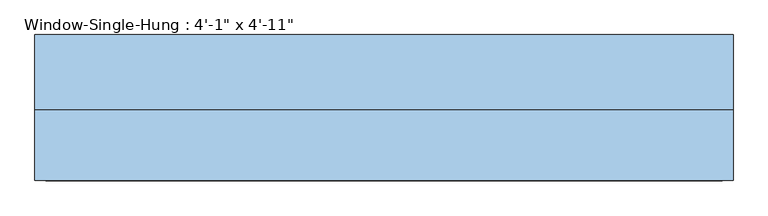
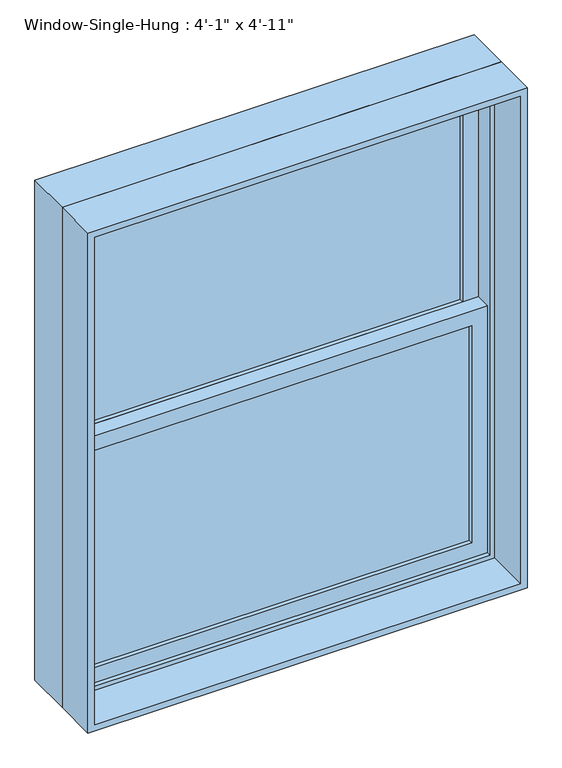
"""IFC4 building model written with IfcOpenShell, lengths in millimetres: window geometry."""

import ifcopenshell
import ifcopenshell.guid

model = None  # the IFC model being written
_history = None  # IfcOwnerHistory: only IFC2X3 demands one
_inside = {}  # id of a spatial element -> (the spatial element, [elements in it])
_under = {}  # id of a project, library or spatial element -> (it, [spatial elements below it])
_declared = {}  # id of a project -> (the project, [libraries it declares])
_typed = {}  # id of a type object -> (the type object, [elements of that type])
_made_of = {}  # id of a material, layer set ... -> (it, [elements and type objects made of it])


def new_model(schema):
    """Start an empty IFC model of exactly this schema.

    Asked for "IFC4X3", IfcOpenShell would pick the latest addendum, in which some entities
    have other attributes; the version numbers below select the first issue.
    IFC2X3 requires an IfcOwnerHistory on every rooted entity: one is made here for all.
    """
    global model, _history
    if schema == "IFC4X3":
        model = ifcopenshell.file(schema_version=(4, 3, 0, 0))
    else:
        model = ifcopenshell.file(schema=schema)
    _inside.clear()
    _under.clear()
    _declared.clear()
    _typed.clear()
    _made_of.clear()
    _history = None
    if model.schema == "IFC2X3":
        org = make("IfcOrganization", Name="unknown")
        user = make(
            "IfcPersonAndOrganization",
            ThePerson=make("IfcPerson", FamilyName="unknown"),
            TheOrganization=org,
        )
        app = make(
            "IfcApplication",
            ApplicationDeveloper=org,
            Version="unknown",
            ApplicationFullName="unknown",
            ApplicationIdentifier="unknown",
        )
        _history = make(
            "IfcOwnerHistory",
            OwningUser=user,
            OwningApplication=app,
            ChangeAction="ADDED",
            CreationDate=0,
        )
    return model


def make(cls, **values):
    """One entity of the class cls with the attributes given. An attribute that is None is left unset."""
    return model.create_entity(
        cls, **{name: value for name, value in values.items() if value is not None}
    )


def rooted(cls, **values):
    """An entity with a GlobalId (a new one), such as an element, a storey or a relation."""
    return make(cls, GlobalId=ifcopenshell.guid.new(), OwnerHistory=_history, **values)


def si_unit(unit_type, name, prefix=None):
    """IfcSIUnit, for example si_unit("LENGTHUNIT", "METRE", prefix="MILLI")."""
    return make("IfcSIUnit", UnitType=unit_type, Prefix=prefix, Name=name)


def assignment(units):
    """IfcUnitAssignment: the units of a project."""
    return None if units is None else make("IfcUnitAssignment", Units=units)


def point(xyz):
    """IfcCartesianPoint."""
    return None if xyz is None else make("IfcCartesianPoint", Coordinates=xyz)


def direction(xyz):
    """IfcDirection."""
    return None if xyz is None else make("IfcDirection", DirectionRatios=xyz)


def frame(location, z_axis=None, x_axis=None):
    """IfcAxis2Placement3D, a coordinate frame: its origin and axes. An axis left out is left unset."""
    return make(
        "IfcAxis2Placement3D",
        Location=point(location),
        Axis=direction(z_axis),
        RefDirection=direction(x_axis),
    )


def origin():
    """The frame at (0, 0, 0) with its axes left unset."""
    return frame((0.0, 0.0, 0.0))


def place(relative_to, where):
    """IfcLocalPlacement: puts the frame where relative to a parent placement (None: the world)."""
    return make(
        "IfcLocalPlacement", PlacementRelTo=relative_to, RelativePlacement=where
    )


def context(
    kind, dimensions, precision=None, world=None, true_north=None, identifier=None
):
    """IfcGeometricRepresentationContext, for example the 3D "Model" context."""
    return make(
        "IfcGeometricRepresentationContext",
        ContextIdentifier=identifier,
        ContextType=kind,
        CoordinateSpaceDimension=dimensions,
        Precision=precision,
        WorldCoordinateSystem=world,
        TrueNorth=true_north,
    )


def project(units=None, contexts=None):
    """IfcProject with its units and contexts."""
    return rooted(
        "IfcProject",
        Name="project",
        RepresentationContexts=contexts,
        UnitsInContext=assignment(units),
    )


def spatial(cls, under=None, at=None, **own):
    """A site, building, storey or space (cls), placed at a placement, below another one or the project."""
    s = rooted(cls, ObjectPlacement=at, **own)
    if under is not None:
        _under.setdefault(under.id(), (under, []))[1].append(s)
    return s


def polyline(points):
    """IfcPolyline through the points."""
    return make("IfcPolyline", Points=[point(p) for p in points])


def outline(outer, holes=None, kind="AREA"):
    """IfcArbitraryClosedProfileDef: a profile drawn as a closed curve; with holes, ...WithVoids."""
    if holes is None:
        return make("IfcArbitraryClosedProfileDef", ProfileType=kind, OuterCurve=outer)
    return make(
        "IfcArbitraryProfileDefWithVoids",
        ProfileType=kind,
        OuterCurve=outer,
        InnerCurves=holes,
    )


def extrude(swept, where, along, depth):
    """IfcExtrudedAreaSolid: the profile swept, set in the frame where, extruded along a direction by depth."""
    return make(
        "IfcExtrudedAreaSolid",
        SweptArea=swept,
        Position=where,
        ExtrudedDirection=direction(along),
        Depth=depth,
    )


def shape(context_of_items, identifier, shape_type, items):
    """IfcShapeRepresentation: the items that make up one representation, for example the "Body"."""
    return make(
        "IfcShapeRepresentation",
        ContextOfItems=context_of_items,
        RepresentationIdentifier=identifier,
        RepresentationType=shape_type,
        Items=items,
    )


def source(mapping_origin, context_of_items, identifier, shape_type, items):
    """IfcRepresentationMap: a shape defined once, which mapped items show again and again."""
    return make(
        "IfcRepresentationMap",
        MappingOrigin=mapping_origin,
        MappedRepresentation=shape(context_of_items, identifier, shape_type, items),
    )


def transform(
    local_origin,
    x_axis=None,
    y_axis=None,
    z_axis=None,
    scale=None,
    scale2=None,
    scale3=None,
    uniform=True,
):
    """IfcCartesianTransformationOperator3D, or its non-uniform kind. x_axis, y_axis, z_axis: its Axis1, 2, 3."""
    if uniform:
        return make(
            "IfcCartesianTransformationOperator3D",
            Axis1=direction(x_axis),
            Axis2=direction(y_axis),
            LocalOrigin=point(local_origin),
            Scale=scale,
            Axis3=direction(z_axis),
        )
    return make(
        "IfcCartesianTransformationOperator3DnonUniform",
        Axis1=direction(x_axis),
        Axis2=direction(y_axis),
        LocalOrigin=point(local_origin),
        Scale=scale,
        Axis3=direction(z_axis),
        Scale2=scale2,
        Scale3=scale3,
    )


def mapped(mapping_source, mapping_target):
    """IfcMappedItem: shows the shape of a source again, moved by a transform."""
    return make(
        "IfcMappedItem", MappingSource=mapping_source, MappingTarget=mapping_target
    )


def made_of(thing, what):
    """Note that an element or type object is made of a material, layer set ...; save() writes the relation."""
    if what is not None:
        _made_of.setdefault(what.id(), (what, []))[1].append(thing)
    return thing


def element(
    cls,
    number,
    at=None,
    inside=None,
    cuts=None,
    type_object=None,
    material=None,
    context=None,
    identifier="Body",
    shape_type=None,
    held_by="IfcProductDefinitionShape",
    body=None,
    shapes=None,
    **own,
):
    """One element of the class cls, such as IfcWall. Its Tag is "e" and its number.

    at: its placement. inside: the storey or other place that contains it. cuts: it is an
    opening in that element (IfcRelVoidsElement). A single representation is given by context,
    identifier, shape_type and body (its items); several are given by shapes. held_by: the class
    of the entity that holds the representations. save() writes the other relations.
    """
    e = rooted(cls, Tag="e%d" % number, ObjectPlacement=at, **own)
    if body is not None:
        shapes = [shape(context, identifier, shape_type, body)]
    if shapes is not None:
        e.Representation = make(held_by, Representations=shapes)
    if inside is not None:
        _inside.setdefault(inside.id(), (inside, []))[1].append(e)
    if cuts is not None:
        rooted(
            "IfcRelVoidsElement", RelatingBuildingElement=cuts, RelatedOpeningElement=e
        )
    if type_object is not None:
        _typed.setdefault(type_object.id(), (type_object, []))[1].append(e)
    return made_of(e, material)


def aggregate(whole, parts):
    """IfcRelAggregates: a whole, such as a stair, and the parts it consists of."""
    return rooted("IfcRelAggregates", RelatingObject=whole, RelatedObjects=parts)


def save(model, path):
    """Write the relations noted so far, then the file.

    IfcRelAggregates (storeys below a building ...), IfcRelContainedInSpatialStructure (elements
    in a storey), IfcRelDefinesByType, IfcRelAssociatesMaterial and IfcRelDeclares: one each for
    every whole, place, type object, material and project.
    """
    for whole, parts in _under.values():
        aggregate(whole, parts)
    for where, things in _inside.values():
        rooted(
            "IfcRelContainedInSpatialStructure",
            RelatedElements=things,
            RelatingStructure=where,
        )
    for kind, things in _typed.values():
        rooted("IfcRelDefinesByType", RelatedObjects=things, RelatingType=kind)
    for what, things in _made_of.values():
        rooted("IfcRelAssociatesMaterial", RelatedObjects=things, RelatingMaterial=what)
    for by, libraries in _declared.values():
        rooted("IfcRelDeclares", RelatingContext=by, RelatedDefinitions=libraries)
    model.write(path)


def window_28033f45(model_context):
    return source(origin(), model_context, "Body", "SweptSolid", [
        extrude(outline(polyline([(546.1, 50.8), (546.1, 44.45), (-546.1, 44.45), (-546.1, 50.8), (546.1, 50.8)])), frame((0.0, 0.0, 990.6), z_axis=(0.0, 0.0, 1.0), x_axis=(1.0, 0.0, 0.0)), (0.0, 0.0, 1.0), 650.875),
        extrude(outline(polyline([(-546.1, 38.1), (546.1, 38.1), (546.1, 31.75), (-546.1, 31.75), (-546.1, 38.1)])), frame((0.0, 0.0, 990.6), z_axis=(0.0, 0.0, 1.0), x_axis=(1.0, 0.0, 0.0)), (0.0, 0.0, 1.0), 650.875),
        extrude(outline(polyline([(546.1, 95.25), (546.1, 88.9), (-546.1, 88.9), (-546.1, 95.25), (546.1, 95.25)])), frame((0.0, 0.0, 1685.925), z_axis=(0.0, 0.0, 1.0), x_axis=(1.0, 0.0, 0.0)), (0.0, 0.0, 1.0), 650.875),
        extrude(outline(polyline([(-546.1, 82.55), (546.1, 82.55), (546.1, 76.2), (-546.1, 76.2), (-546.1, 82.55)])), frame((0.0, 0.0, 1685.925), z_axis=(0.0, 0.0, 1.0), x_axis=(1.0, 0.0, 0.0)), (0.0, 0.0, 1.0), 650.875),
        extrude(outline(polyline([(1685.925, -590.55), (946.15, -590.55), (946.15, 590.55), (1685.925, 590.55), (1685.925, -590.55)]), holes=[polyline([(1641.475, 546.1), (990.6, 546.1), (990.6, -546.1), (1641.475, -546.1), (1641.475, 546.1)])]), frame((0.0, 19.05, 0.0), z_axis=(0.0, 1.0, 0.0), x_axis=(0.0, 0.0, 1.0)), (0.0, 0.0, 1.0), 44.45),
        extrude(outline(polyline([(2381.25, -590.55), (1641.475, -590.55), (1641.475, 590.55), (2381.25, 590.55), (2381.25, -590.55)]), holes=[polyline([(2336.8, 546.1), (1685.925, 546.1), (1685.925, -546.1), (2336.8, -546.1), (2336.8, 546.1)])]), frame((0.0, 63.5, 0.0), z_axis=(0.0, 1.0, 0.0), x_axis=(0.0, 0.0, 1.0)), (0.0, 0.0, 1.0), 44.45),
        extrude(outline(polyline([(2413.0, -622.3), (914.4, -622.3), (914.4, 622.3), (2413.0, 622.3), (2413.0, -622.3)]), holes=[polyline([(2381.25, 590.55), (946.15, 590.55), (946.15, -590.55), (2381.25, -590.55), (2381.25, 590.55)])]), frame((0.0, 6.35, 0.0), z_axis=(0.0, 1.0, 0.0), x_axis=(0.0, 0.0, 1.0)), (0.0, 0.0, 1.0), 133.35),
        extrude(outline(polyline([(2413.0, 622.3), (2413.0, -622.3), (914.4, -622.3), (914.4, 622.3), (2413.0, 622.3)]), holes=[polyline([(2393.95, 603.25), (933.45, 603.25), (933.45, -603.25), (2393.95, -603.25), (2393.95, 603.25)])]), frame((0.0, -120.65, 0.0), z_axis=(0.0, 1.0, 0.0), x_axis=(0.0, 0.0, 1.0)), (0.0, 0.0, 1.0), 127.0),
    ])


if __name__ == "__main__":
    model = new_model("IFC4")
    model_context = context("Model", 3, world=origin())
    ifc_project = project(units=[si_unit("LENGTHUNIT", "METRE", prefix="MILLI")], contexts=[model_context])
    site = spatial("IfcSite", under=ifc_project)
    building = spatial("IfcBuilding", under=site)
    placement = place(None, origin())
    window_shape = window_28033f45(model_context)
    element("IfcWindow", 1, ObjectType="Window-Single-Hung : 4'-1\" x 4'-11\"", at=placement, inside=building, context=model_context, shape_type="MappedRepresentation", body=[
        mapped(window_shape, transform((0.0, 0.0, 0.0), x_axis=(1.0, 0.0, 0.0), y_axis=(0.0, 1.0, 0.0), z_axis=(0.0, 0.0, 1.0))),
    ])
    save(model, "model.ifc")

# Revit data of these elements
# Type "Window-Single-Hung : 4'-1\" x 4'-11\""
#   Type Mark = "20"
#   Fire Rating = "0.5h"
#   Construction Type Id = "DG-DR"
#   Assembly Code = "B2020100"
#   Analytic Construction = "Double glazing - domestic"
#   Wall Thickness [instance default] = 0' - 6"
#   Window Inset [instance default] = 0' - 0"
#   Visual Light Transmittance = 0.81
#   Thermal Resistance (R) = 0.319569 (m²·K)/W
#   Solar Heat Gain Coefficient = 0.76
#   Muntin Width = 3' - 7"
#   Muntin Height = 2' - 1 5/8"
#   Interior Wall Closure [instance default] = 0' - 1 1/2"
#   Rough Width = 4' - 1 1/2"
#   Rough Height = 4' - 11 1/2"
#   Frame Extension [instance default] = 0' - 1 1/4"
#   Exterior Wall Closure [instance default] = 0' - 0 1/2"
#   Extension Jamb [instance default] = 0' - 1 1/2"
#   Heat Transfer Coefficient (U) = 3.12929 W/(m²·K)
#   Height = 4' - 11"
#   Width = 4' - 1"
#   Top Muntin Visibility = yes
#   Indicator Visibility [instance default] = yes
#   Extension Jamb Visibility [instance default] = yes
#   Interior Trim Visibility [instance default] = yes
#   Exterior Trim Visibility [instance default] = yes
#   Bottom Muntin Visibility = yes
#   Muntin Pattern = Muntin Pattern_2x2 : Muntin Pattern_2x2
#   Interior Trim Material = Wood - Stained
#   Interior Trim = Trim-Window-Interior-Flat : Picture Frame
#   Exterior Trim Material = Clad - White
#   Exterior Trim = Trim-Window-Exterior-Flat : with Sill
#   Glass Panel Material = Glass
#   Exterior Frame Material = Clad - White
#   Interior Frame Material = Wood - Stained
#   Wall Closure = (empty or 0)
# Element 1 (IfcWindow, "Window-Single-Hung : 4'-1\" x 4'-11\"")
#   Wall Thickness = 0' - 9 1/2"
#   Extension Jamb = 0' - 5"
#   Materials on its faces: "Wood - Stained", "Glass", "Clad - White"
# Materials
#   "Wood - Stained": class "Wood", colour RGB 224 178 126, transparency 0, Cost = 0
#   "Clad - White": class "Wood", colour RGB 242 242 238, transparency 0, Cost = 0
#   "Glass": class "Glass", colour RGB 0 128 192, transparency 0.75, Description = "Soda Lime Glass", Cost = 0
